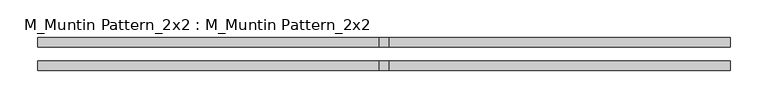
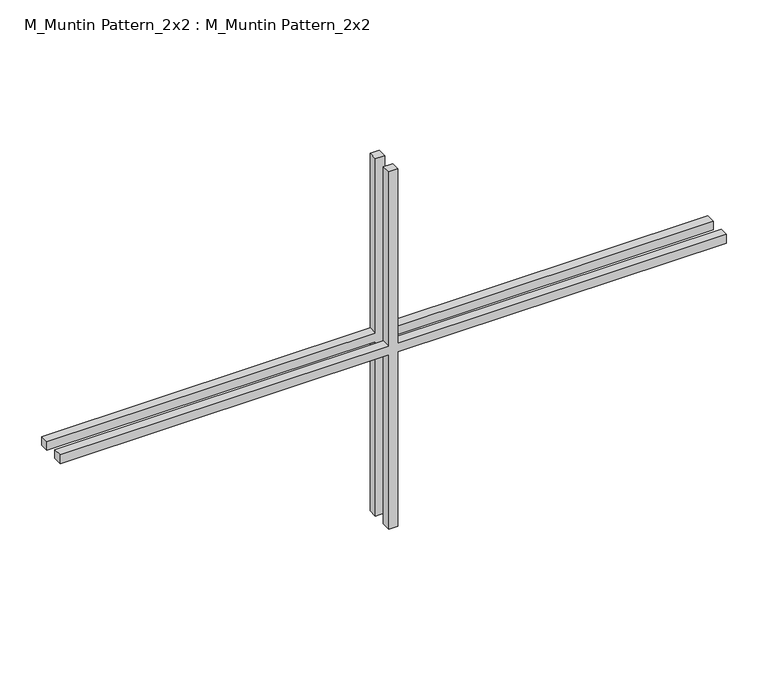
"""IFC4 building model written with IfcOpenShell, lengths in millimetres: proxy geometry, M_Muntin Pattern_2x2 : M_Muntin Pattern_2x2."""

from ifc_helpers import new_model, si_unit, frame, origin, place, context, project, spatial, polyline, outline, extrude, source, transform, mapped, element, save


def m_muntin_pattern_2x2_m_muntin_pattern_2x2_17b20c59(model_context):
    return source(origin(), model_context, "Body", "SweptSolid", [
        extrude(outline(polyline([(268.25, -6.35), (268.25, -461.9), (255.55, -461.9), (255.55, -6.35), (0.0, -6.35), (0.0, 6.35), (255.55, 6.35), (255.55, 461.9), (268.25, 461.9), (268.25, 6.35), (523.8, 6.35), (523.8, -6.35), (268.25, -6.35)])), frame((0.0, -22.225, 0.0), z_axis=(0.0, 1.0, 0.0), x_axis=(0.0, 0.0, 1.0)), (0.0, 0.0, 1.0), 12.7),
        extrude(outline(polyline([(268.25, -6.35), (268.25, -461.9), (255.55, -461.9), (255.55, -6.35), (0.0, -6.35), (0.0, 6.35), (255.55, 6.35), (255.55, 461.9), (268.25, 461.9), (268.25, 6.35), (523.8, 6.35), (523.8, -6.35), (268.25, -6.35)])), frame((0.0, 9.525, 0.0), z_axis=(0.0, 1.0, 0.0), x_axis=(0.0, 0.0, 1.0)), (0.0, 0.0, 1.0), 12.7),
    ])


if __name__ == "__main__":
    model = new_model("IFC4")
    model_context = context("Model", 3, world=origin())
    ifc_project = project(units=[si_unit("LENGTHUNIT", "METRE", prefix="MILLI")], contexts=[model_context])
    site = spatial("IfcSite", under=ifc_project)
    building = spatial("IfcBuilding", under=site)
    placement = place(None, origin())
    m_muntin_pattern_2x2_m_muntin_pattern_2x2_shape = m_muntin_pattern_2x2_m_muntin_pattern_2x2_17b20c59(model_context)
    element("IfcBuildingElementProxy", 1, Name="M_Muntin Pattern_2x2 : M_Muntin Pattern_2x2", ObjectType="M_Muntin Pattern_2x2 : M_Muntin Pattern_2x2", at=placement, inside=building, context=model_context, shape_type="MappedRepresentation", body=[
        mapped(m_muntin_pattern_2x2_m_muntin_pattern_2x2_shape, transform((0.0, 0.0, 0.0), x_axis=(1.0, 0.0, 0.0), y_axis=(0.0, 1.0, 0.0), z_axis=(0.0, 0.0, 1.0))),
    ])
    save(model, "model.ifc")

# Revit data of these elements
# Type "M_Muntin Pattern_2x2 : M_Muntin Pattern_2x2"
#   Width [instance default] = 1200 mm
#   Thickness = 12.7 mm
#   Height [instance default] = 1200 mm
#   Distance = 19.05 mm
#   Interior Material [instance default] = none
#   Exterior Material [instance default] = none
#   Default Elevation = 0
# Element 1 (IfcBuildingElementProxy, "M_Muntin Pattern_2x2 : M_Muntin Pattern_2x2")
#   Width = 923.8 mm
#   Height = 523.8 mm
#   Interior Material = Wood - Stained
#   Exterior Material = Clad - White
#   Materials on its faces: "Clad - White", "Wood - Stained"
# Materials
#   "Clad - White": class "Wood", colour RGB 245 245 243, transparency 0, Cost = 0
#   "Wood - Stained": class "Wood", colour RGB 173 132 96, transparency 0, Cost = 0
